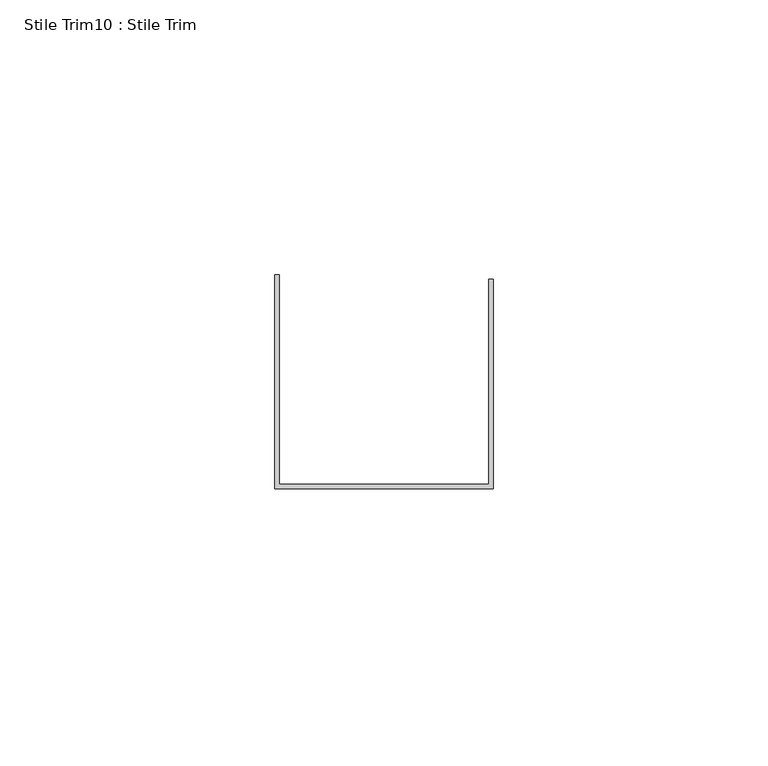
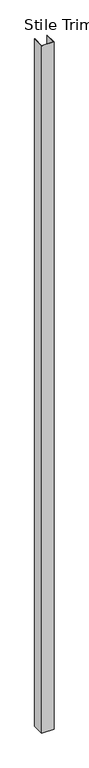
"""IFC4 building model written with IfcOpenShell, lengths in millimetres: proxy geometry, Stile Trim10 : Stile Trim."""

from ifc_helpers import new_model, si_unit, frame, origin, place, context, project, spatial, polyline, outline, extrude, source, transform, mapped, element, save


def stile_trim10_stile_trim_2fa88a95(model_context):
    return source(origin(), model_context, "Body", "SweptSolid", [
        extrude(outline(polyline([(587327.0060739, -535202.3537841), (587327.0060739, -535163.4663841), (587327.7934739, -535163.4663841), (587327.7934739, -535201.5663841), (587365.8934739, -535201.5663841), (587365.8934739, -535164.2537841), (587366.6808739, -535164.2537841), (587366.6808739, -535202.3537841), (587327.0060739, -535202.3537841)])), frame((0.0, 0.0, 50.8), z_axis=(0.0, 0.0, 1.0), x_axis=(1.0, 0.0, 0.0)), (0.0, 0.0, 1.0), 2350.3929688),
    ])


if __name__ == "__main__":
    model = new_model("IFC4")
    model_context = context("Model", 3, world=origin())
    ifc_project = project(units=[si_unit("LENGTHUNIT", "METRE", prefix="MILLI")], contexts=[model_context])
    site = spatial("IfcSite", under=ifc_project)
    building = spatial("IfcBuilding", under=site)
    placement = place(None, origin())
    stile_trim10_stile_trim_shape = stile_trim10_stile_trim_2fa88a95(model_context)
    element("IfcBuildingElementProxy", 1, Name="Stile Trim10 : Stile Trim", ObjectType="Stile Trim10 : Stile Trim", at=placement, inside=building, context=model_context, shape_type="MappedRepresentation", body=[
        mapped(stile_trim10_stile_trim_shape, transform((0.0, 0.0, 0.0), x_axis=(1.0, 0.0, 0.0), y_axis=(0.0, 1.0, 0.0), z_axis=(0.0, 0.0, 1.0))),
    ])
    save(model, "model.ifc")

# Revit data of these elements
# Element 1 (IfcBuildingElementProxy, "Stile Trim10 : Stile Trim")
#   Materials on its faces: "EDGE TRIM BY MTL PANEL MFR."
# Materials
#   "EDGE TRIM BY MTL PANEL MFR.": class "Generic", colour RGB 239 242 240, transparency 0, Cost = 0
